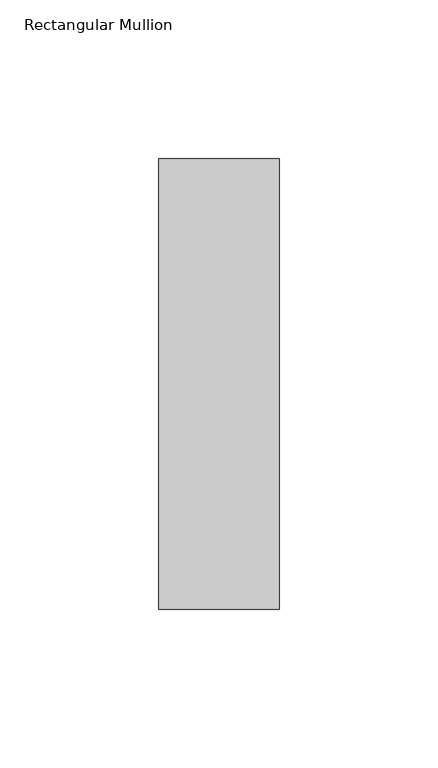
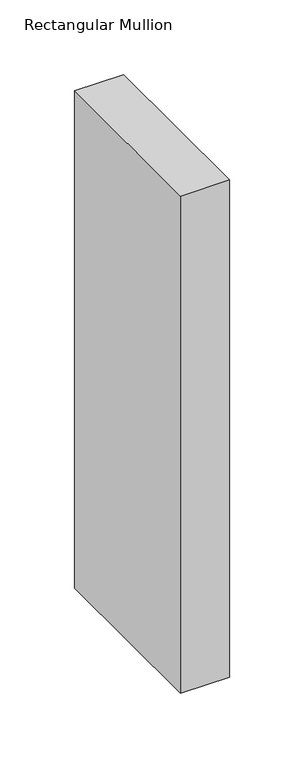
"""IFC4 building model written with IfcOpenShell, lengths in millimetres: member geometry, Rectangular Mullion : NLRS_21_CWM_hsb-regel 38x142_gen_rsf."""

from ifc_helpers import new_model, si_unit, frame, origin, place, context, project, spatial, polyline, outline, extrude, source, transform, mapped, element, save


def rectangular_mullion_51268c3e(model_context):
    return source(origin(), model_context, "Body", "SweptSolid", [
        extrude(outline(polyline([(0.0, -71.0), (-38.0, -71.0), (-38.0, 71.0), (0.0, 71.0), (0.0, -71.0)])), frame((0.0, 0.0, -407.0), z_axis=(0.0, 0.0, 1.0), x_axis=(1.0, 0.0, 0.0)), (0.0, 0.0, 1.0), 407.0),
    ])


if __name__ == "__main__":
    model = new_model("IFC4")
    model_context = context("Model", 3, world=origin())
    ifc_project = project(units=[si_unit("LENGTHUNIT", "METRE", prefix="MILLI")], contexts=[model_context])
    site = spatial("IfcSite", under=ifc_project)
    building = spatial("IfcBuilding", under=site)
    placement = place(None, origin())
    rectangular_mullion_shape = rectangular_mullion_51268c3e(model_context)
    element("IfcMember", 1, ObjectType="Rectangular Mullion : NLRS_21_CWM_hsb-regel 38x142_gen_rsf", at=placement, inside=building, context=model_context, shape_type="MappedRepresentation", body=[
        mapped(rectangular_mullion_shape, transform((0.0, 0.0, 0.0), x_axis=(1.0, 0.0, 0.0), y_axis=(0.0, 1.0, 0.0), z_axis=(0.0, 0.0, 1.0))),
    ])
    save(model, "model.ifc")

# Revit data of these elements
# Type "Rectangular Mullion : NLRS_21_CWM_hsb-regel 38x142_gen_rsf"
#   Export Type to IFC As = "IfcWall"
#   Type IfcGUID = "07M7mRoiH1CR8m_RSKIwpF"
#   Assembly Code = "21.10"
#   built-in parameter 1007322 = 0.465879 (stored number, unit not read)
#   built-in parameter 1007321 = 0.062336 (stored number, unit not read)
#   built-in parameter 1007320 = 0.062336 (stored number, unit not read)
# Element 1 (IfcMember, "Rectangular Mullion : NLRS_21_CWM_hsb-regel 38x142_gen_rsf")
#   Materials on its faces: "NLRS_i2_hout naaldhout vuren_gen_rsf"
# Materials
#   "NLRS_i2_hout naaldhout vuren_gen_rsf": class "I - Hout", colour RGB 234 199 147, transparency 0, Keynote = "i2", Manufacturer = "Revit Standards Foundation", URL = "www.revitstandards.org", Description = "hout vuren", Cost = 0
